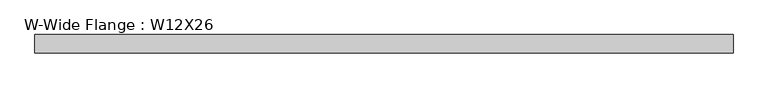
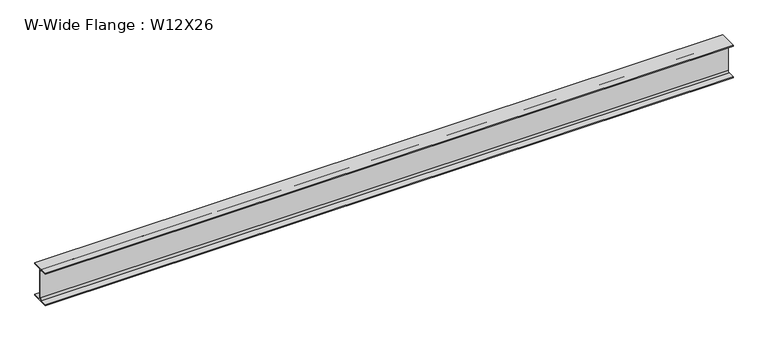
"""IFC4 building model written with IfcOpenShell, lengths in millimetres: beam geometry, W-Wide Flange : W12X26."""

from ifc_helpers import new_model, si_unit, point, frame, frame_2d, origin, place, context, project, spatial, polyline, circle_curve, trimmed, segment, composite_curve, outline, extrude, source, transform, mapped, element, save


def w_wide_flange_w12x26_b6252b85(model_context):
    return source(origin(), model_context, "Body", "SweptSolid", [
        extrude(outline(composite_curve([segment(polyline([(82.4011719, -145.5539063), (82.4011719, -155.178125), (-82.4011719, -155.178125), (-82.4011719, -145.5539063), (-20.2902344, -145.5539063)]), True, "CONTINUOUS"), segment(trimmed(circle_curve(frame_2d((-20.2902344, -128.190625)), 17.3632812), [point((-20.2902344, -145.5539063))], [point((-2.9269531, -128.190625))], True, "CARTESIAN"), True, "CONTINUOUS"), segment(polyline([(-2.9269531, -128.190625), (-2.9269531, 128.190625)]), True, "CONTINUOUS"), segment(trimmed(circle_curve(frame_2d((-20.2902344, 128.190625)), 17.3632812), [point((-2.9269531, 128.190625))], [point((-20.2902344, 145.5539062))], True, "CARTESIAN"), True, "CONTINUOUS"), segment(polyline([(-20.2902344, 145.5539062), (-82.4011719, 145.5539062), (-82.4011719, 155.178125), (82.4011719, 155.178125), (82.4011719, 145.5539062), (20.2902344, 145.5539062)]), True, "CONTINUOUS"), segment(trimmed(circle_curve(frame_2d((20.2902344, 128.190625)), 17.3632812), [point((20.2902344, 145.5539062))], [point((2.9269531, 128.190625))], True, "CARTESIAN"), True, "CONTINUOUS"), segment(polyline([(2.9269531, 128.190625), (2.9269531, -128.190625)]), True, "CONTINUOUS"), segment(trimmed(circle_curve(frame_2d((20.2902344, -128.190625)), 17.3632812), [point((2.9269531, -128.190625))], [point((20.2902344, -145.5539063))], True, "CARTESIAN"), True, "CONTINUOUS"), segment(polyline([(20.2902344, -145.5539063), (82.4011719, -145.5539063)]), True, "CONTINUOUS")], self_intersect=False)), frame((-3105.2988281, 0.0, 0.0), z_axis=(1.0, 0.0, 0.0), x_axis=(0.0, 1.0, 0.0)), (0.0, 0.0, 1.0), 6210.5976562),
    ])


if __name__ == "__main__":
    model = new_model("IFC4")
    model_context = context("Model", 3, world=origin())
    ifc_project = project(units=[si_unit("LENGTHUNIT", "METRE", prefix="MILLI")], contexts=[model_context])
    site = spatial("IfcSite", under=ifc_project)
    building = spatial("IfcBuilding", under=site)
    placement = place(None, origin())
    w_wide_flange_w12x26_shape = w_wide_flange_w12x26_b6252b85(model_context)
    element("IfcBeam", 1, ObjectType="W-Wide Flange : W12X26", at=placement, inside=building, context=model_context, shape_type="MappedRepresentation", body=[
        mapped(w_wide_flange_w12x26_shape, transform((0.0, 0.0, 0.0), x_axis=(1.0, 0.0, 0.0), y_axis=(0.0, 1.0, 0.0), z_axis=(0.0, 0.0, 1.0))),
    ])
    save(model, "model.ifc")

# Revit data of these elements
# Type "W-Wide Flange : W12X26"
#   Assembly Code = "B10"
#   W = 26
#   Length [instance default] = 5' - 0"
#   bf = 0' - 6 125/256"
#   d = 1' - 0 7/32"
#   k = 0' - 1 1/16"
#   k2 = 0' - 0 175/256"
#   tf = 0' - 0 97/256"
#   tw = 0' - 0 59/256"
#   A = 0.053125 SF
#   Structural Material [instance default] = none
# Element 1 (IfcBeam, "W-Wide Flange : W12X26")
#   Structural Material = Dark metal
#   Materials on its faces: "Dark metal"
# Materials
#   "Dark metal": class "Generic", colour RGB 44 29 29, transparency 0, Cost = 0
